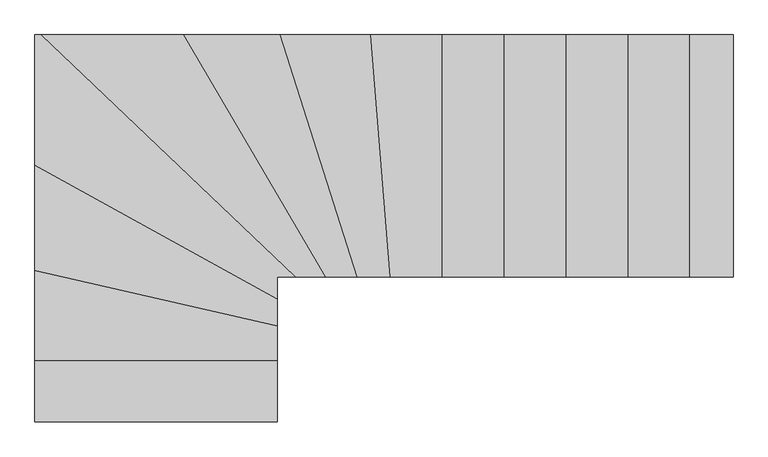
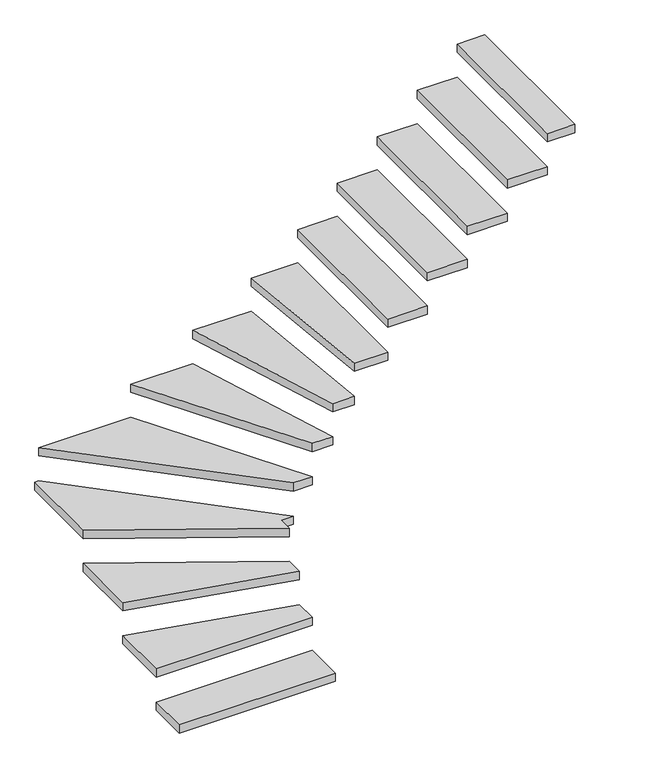
"""IFC4 building model written with IfcOpenShell, lengths in millimetres: stair geometry,   151260 :   151260."""

from ifc_helpers import new_model, si_unit, frame, origin, place, context, project, spatial, polyline, outline, extrude, source, transform, mapped, element, save


def stair_4856ba97(model_context):
    return source(origin(), model_context, "Body", "SweptSolid", [
        extrude(outline(polyline([(159177.7593015, 39074.7962965), (160077.7593015, 39074.7962965), (160077.7593015, 38844.7962965), (159177.7593015, 38844.7962965), (159177.7593015, 39074.7962965)])), frame((0.0, 0.0, 3482.1428571), z_axis=(0.0, 0.0, 1.0), x_axis=(1.0, 0.0, 0.0)), (0.0, 0.0, 1.0), 50.0),
        extrude(outline(polyline([(159177.7593015, 39407.7634868), (160077.7593015, 39201.8291061), (160077.7593015, 39074.7962965), (159177.7593015, 39074.7962965), (159177.7593015, 39407.7634868)])), frame((0.0, 0.0, 3684.2857143), z_axis=(0.0, 0.0, 1.0), x_axis=(1.0, 0.0, 0.0)), (0.0, 0.0, 1.0), 50.0),
        extrude(outline(polyline([(159177.7593015, 39801.0914939), (160077.7593015, 39301.7193734), (160077.7593015, 39201.8291061), (159177.7593015, 39407.7634868), (159177.7593015, 39801.0914939)])), frame((0.0, 0.0, 3886.4285714), z_axis=(0.0, 0.0, 1.0), x_axis=(1.0, 0.0, 0.0)), (0.0, 0.0, 1.0), 50.0),
        extrude(outline(polyline([(159177.7593015, 40284.7962965), (159200.4297176, 40284.7962965), (160147.7593015, 39384.7962965), (160077.7593015, 39384.7962965), (160077.7593015, 39301.7193734), (159177.7593015, 39801.0914939), (159177.7593015, 40284.7962965)])), frame((0.0, 0.0, 4088.5714286), z_axis=(0.0, 0.0, 1.0), x_axis=(1.0, 0.0, 0.0)), (0.0, 0.0, 1.0), 50.0),
        extrude(outline(polyline([(159730.1980238, 40284.7962965), (160258.7713888, 39384.7962965), (160147.7593015, 39384.7962965), (159200.4297176, 40284.7962965), (159730.1980238, 40284.7962965)])), frame((0.0, 0.0, 4290.7142857), z_axis=(0.0, 0.0, 1.0), x_axis=(1.0, 0.0, 0.0)), (0.0, 0.0, 1.0), 50.0),
        extrude(outline(polyline([(160089.4284981, 40284.7962965), (160375.293778, 39384.7962965), (160258.7713888, 39384.7962965), (159730.1980238, 40284.7962965), (160089.4284981, 40284.7962965)])), frame((0.0, 0.0, 4492.8571429), z_axis=(0.0, 0.0, 1.0), x_axis=(1.0, 0.0, 0.0)), (0.0, 0.0, 1.0), 50.0),
        extrude(outline(polyline([(160425.6183342, 40284.7962965), (160499.1039419, 39384.7962965), (160375.293778, 39384.7962965), (160089.4284981, 40284.7962965), (160425.6183342, 40284.7962965)])), frame((0.0, 0.0, 4695.0), z_axis=(0.0, 0.0, 1.0), x_axis=(1.0, 0.0, 0.0)), (0.0, 0.0, 1.0), 50.0),
        extrude(outline(polyline([(160692.3611381, 40284.7962965), (160692.3611381, 39384.7962965), (160499.1039419, 39384.7962965), (160425.6183342, 40284.7962965), (160692.3611381, 40284.7962965)])), frame((0.0, 0.0, 4897.1428571), z_axis=(0.0, 0.0, 1.0), x_axis=(1.0, 0.0, 0.0)), (0.0, 0.0, 1.0), 50.0),
        extrude(outline(polyline([(160922.3611381, 40284.7962965), (160922.3611381, 39384.7962965), (160692.3611381, 39384.7962965), (160692.3611381, 40284.7962965), (160922.3611381, 40284.7962965)])), frame((0.0, 0.0, 5099.2857143), z_axis=(0.0, 0.0, 1.0), x_axis=(1.0, 0.0, 0.0)), (0.0, 0.0, 1.0), 50.0),
        extrude(outline(polyline([(161152.3611381, 40284.7962965), (161152.3611381, 39384.7962965), (160922.3611381, 39384.7962965), (160922.3611381, 40284.7962965), (161152.3611381, 40284.7962965)])), frame((0.0, 0.0, 5301.4285714), z_axis=(0.0, 0.0, 1.0), x_axis=(1.0, 0.0, 0.0)), (0.0, 0.0, 1.0), 50.0),
        extrude(outline(polyline([(161382.3611381, 40284.7962965), (161382.3611381, 39384.7962965), (161152.3611381, 39384.7962965), (161152.3611381, 40284.7962965), (161382.3611381, 40284.7962965)])), frame((0.0, 0.0, 5503.5714286), z_axis=(0.0, 0.0, 1.0), x_axis=(1.0, 0.0, 0.0)), (0.0, 0.0, 1.0), 50.0),
        extrude(outline(polyline([(161612.3611381, 40284.7962965), (161612.3611381, 39384.7962965), (161382.3611381, 39384.7962965), (161382.3611381, 40284.7962965), (161612.3611381, 40284.7962965)])), frame((0.0, 0.0, 5705.7142857), z_axis=(0.0, 0.0, 1.0), x_axis=(1.0, 0.0, 0.0)), (0.0, 0.0, 1.0), 50.0),
        extrude(outline(polyline([(161772.7593015, 40284.7962965), (161772.7593015, 39384.7962965), (161612.3611381, 39384.7962965), (161612.3611381, 40284.7962965), (161772.7593015, 40284.7962965)])), frame((0.0, 0.0, 5907.8571429), z_axis=(0.0, 0.0, 1.0), x_axis=(1.0, 0.0, 0.0)), (0.0, 0.0, 1.0), 50.0),
    ])


if __name__ == "__main__":
    model = new_model("IFC4")
    model_context = context("Model", 3, world=origin())
    ifc_project = project(units=[si_unit("LENGTHUNIT", "METRE", prefix="MILLI")], contexts=[model_context])
    site = spatial("IfcSite", under=ifc_project)
    building = spatial("IfcBuilding", under=site)
    placement = place(None, origin())
    stair_shape = stair_4856ba97(model_context)
    element("IfcStair", 1, ObjectType="  151260 :   151260", at=placement, inside=building, context=model_context, shape_type="MappedRepresentation", body=[
        mapped(stair_shape, transform((0.0, 0.0, 0.0), x_axis=(1.0, 0.0, 0.0), y_axis=(0.0, 1.0, 0.0), z_axis=(0.0, 0.0, 1.0))),
    ])
    save(model, "model.ifc")

# Revit data of these elements
# Type "  151260 :   151260"
#   Abrechnungsart = "St"
#   Allright_Bauteil_ID = "0131Tre0659044533"
#   Material = "Stahlbeton"
#   Objektname = "Treppe"
#   NameOverride = " "
#   ThermalTransmittance = 0.0000 BTU/(h·ft²·°F)
#   NosingLength = 0.000 m
#   NumberOfRiser = 14
#   NumberOfTreads = 13
#   RiserHeight = 2.021 m
#   TreadLength = 2.300 m
#   IsExternal = no
#   FireExit = no
#   HandicapAccessible = no
#   HasNonSkidSurface = no
# Element 1 (IfcStair, "  151260 :   151260")
#   Materials on its faces: "weiss"
# Materials
#   "weiss": class "Unassigned", colour RGB 255 255 255, transparency 0
